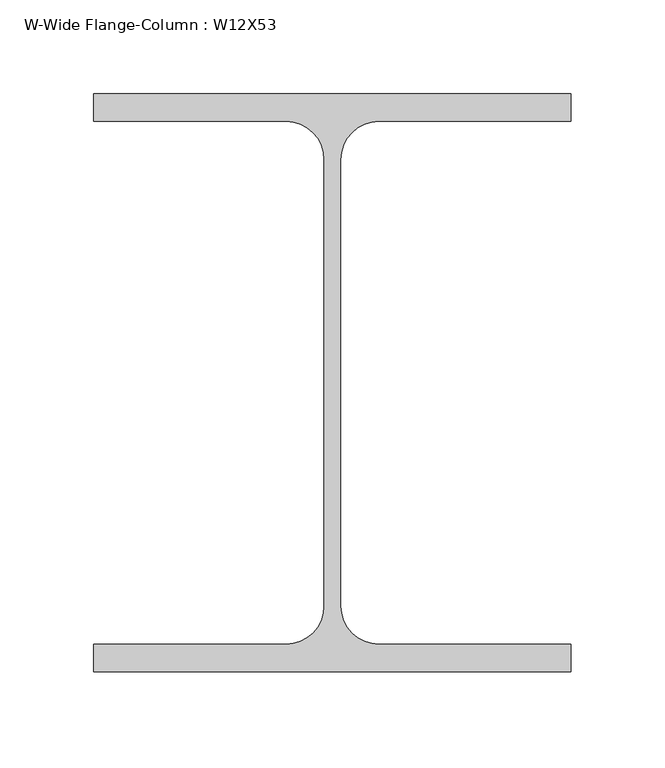
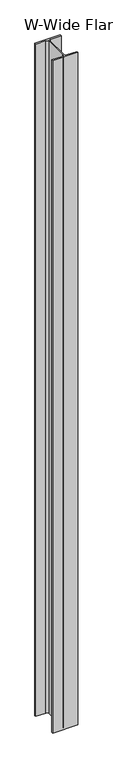
"""IFC4 building model written with IfcOpenShell, lengths in millimetres: column geometry, W-Wide Flange-Column : W12X53."""

from ifc_helpers import new_model, si_unit, point, frame, frame_2d, origin, place, context, project, spatial, polyline, circle_curve, trimmed, segment, composite_curve, outline, extrude, source, transform, mapped, element, save


def w_wide_flange_column_w12x53_9f3dc712(model_context):
    return source(origin(), model_context, "Body", "SweptSolid", [
        extrude(outline(composite_curve([segment(polyline([(127.0, 153.67), (127.0, 139.065), (24.7015, 139.065)]), True, "CONTINUOUS"), segment(trimmed(circle_curve(frame_2d((24.7015, 118.745)), 20.32), [point((24.7015, 139.065))], [point((4.3815, 118.745))], True, "CARTESIAN"), True, "CONTINUOUS"), segment(polyline([(4.3815, 118.745), (4.3815, -118.745)]), True, "CONTINUOUS"), segment(trimmed(circle_curve(frame_2d((24.7015, -118.745)), 20.32), [point((4.3815, -118.745))], [point((24.7015, -139.065))], True, "CARTESIAN"), True, "CONTINUOUS"), segment(polyline([(24.7015, -139.065), (127.0, -139.065), (127.0, -153.67), (-127.0, -153.67), (-127.0, -139.065), (-24.7015, -139.065)]), True, "CONTINUOUS"), segment(trimmed(circle_curve(frame_2d((-24.7015, -118.745)), 20.32), [point((-24.7015, -139.065))], [point((-4.3815, -118.745))], True, "CARTESIAN"), True, "CONTINUOUS"), segment(polyline([(-4.3815, -118.745), (-4.3815, 118.745)]), True, "CONTINUOUS"), segment(trimmed(circle_curve(frame_2d((-24.7015, 118.745)), 20.32), [point((-4.3815, 118.745))], [point((-24.7015, 139.065))], True, "CARTESIAN"), True, "CONTINUOUS"), segment(polyline([(-24.7015, 139.065), (-127.0, 139.065), (-127.0, 153.67), (127.0, 153.67)]), True, "CONTINUOUS")], self_intersect=False)), frame((0.0, 0.0, 8756.65), z_axis=(0.0, 0.0, 1.0), x_axis=(1.0, 0.0, 0.0)), (0.0, 0.0, 1.0), 7146.3296875),
    ])


if __name__ == "__main__":
    model = new_model("IFC4")
    model_context = context("Model", 3, world=origin())
    ifc_project = project(units=[si_unit("LENGTHUNIT", "METRE", prefix="MILLI")], contexts=[model_context])
    site = spatial("IfcSite", under=ifc_project)
    building = spatial("IfcBuilding", under=site)
    placement = place(None, origin())
    w_wide_flange_column_w12x53_shape = w_wide_flange_column_w12x53_9f3dc712(model_context)
    element("IfcColumn", 1, ObjectType="W-Wide Flange-Column : W12X53", at=placement, inside=building, context=model_context, shape_type="MappedRepresentation", body=[
        mapped(w_wide_flange_column_w12x53_shape, transform((0.0, 0.0, 0.0), x_axis=(1.0, 0.0, 0.0), y_axis=(0.0, 1.0, 0.0), z_axis=(0.0, 0.0, 1.0))),
    ])
    save(model, "model.ifc")

# Revit data of these elements
# Type "W-Wide Flange-Column : W12X53"
#   Assembly Code = "B10"
#   W = 53
#   bf = 0' - 10"
#   d = 1' - 0.1"
#   k = 0' - 1 3/8"
#   kr = 0' - 0.8"
#   tf = 0' - 0.575"
#   tw = 0' - 0.345"
#   A = 0.108333 SF
#   Structural Material [instance default] = Steel ASTM A992
# Element 1 (IfcColumn, "W-Wide Flange-Column : W12X53")
#   Materials on its faces: "Steel ASTM A992"
# Materials
#   "Steel ASTM A992": class "Metal", colour RGB 199 199 199, transparency 0, Description = "Structural steel 50ksi", Cost = 0
